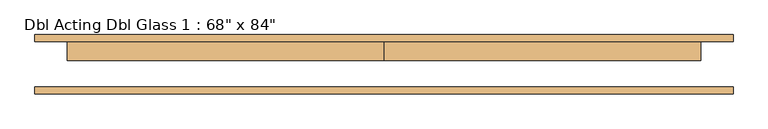
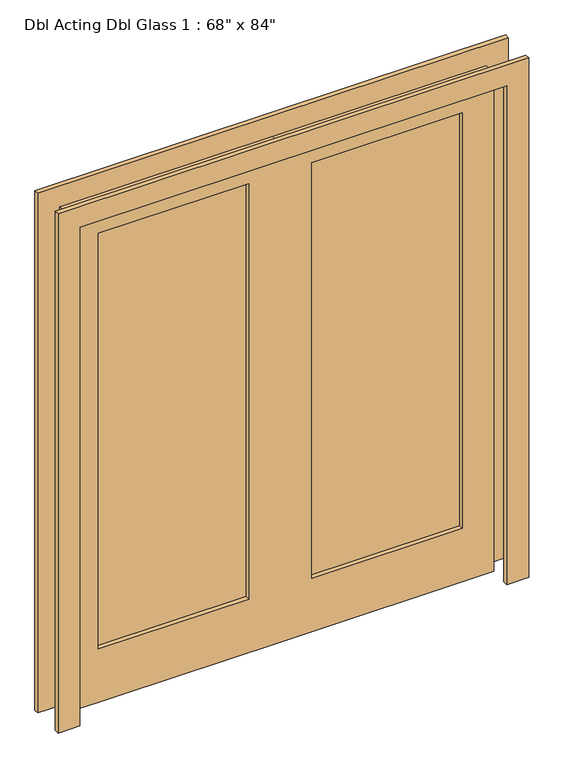
"""IFC4 building model written with IfcOpenShell, lengths in millimetres: door geometry."""

from ifc_helpers import new_model, si_unit, frame, origin, place, context, project, spatial, polyline, outline, extrude, source, transform, mapped, element, save


def door_85c6249d(model_context):
    return source(origin(), model_context, "Body", "SweptSolid", [
        extrude(outline(polyline([(127.0, 68.2625), (736.6, 68.2625), (736.6, 55.5625), (127.0, 55.5625), (127.0, 68.2625)])), frame((0.0, 0.0, 228.6), z_axis=(0.0, 0.0, 1.0), x_axis=(1.0, 0.0, 0.0)), (0.0, 0.0, 1.0), 1778.0),
        extrude(outline(polyline([(-736.6, 68.2625), (-127.0, 68.2625), (-127.0, 55.5625), (-736.6, 55.5625), (-736.6, 68.2625)])), frame((0.0, 0.0, 228.6), z_axis=(0.0, 0.0, 1.0), x_axis=(1.0, 0.0, 0.0)), (0.0, 0.0, 1.0), 1778.0),
        extrude(outline(polyline([(2133.6, 0.0), (2133.6, -863.6), (0.0, -863.6), (0.0, 0.0), (0.0, 863.6), (2133.6, 863.6), (2133.6, 0.0)]), holes=[polyline([(2006.6, 127.0), (2006.6, 736.6), (228.6, 736.6), (228.6, 127.0), (2006.6, 127.0)]), polyline([(2006.6, -127.0), (228.6, -127.0), (228.6, -736.6), (2006.6, -736.6), (2006.6, -127.0)])]), frame((0.0, 36.5125, 0.0), z_axis=(0.0, 1.0, 0.0), x_axis=(0.0, 0.0, 1.0)), (0.0, 0.0, 1.0), 50.8),
        extrude(outline(polyline([(2133.6, -863.6), (2133.6, 863.6), (0.0, 863.6), (0.0, 952.5), (2222.5, 952.5), (2222.5, -952.5), (0.0, -952.5), (0.0, -863.6), (2133.6, -863.6)])), frame((0.0, -55.5625, 0.0), z_axis=(0.0, 1.0, 0.0), x_axis=(0.0, 0.0, 1.0)), (0.0, 0.0, 1.0), 19.05),
        extrude(outline(polyline([(2133.6, -863.6), (2133.6, 863.6), (0.0, 863.6), (0.0, 952.5), (2222.5, 952.5), (2222.5, -952.5), (0.0, -952.5), (0.0, -863.6), (2133.6, -863.6)])), frame((0.0, 87.3125, 0.0), z_axis=(0.0, 1.0, 0.0), x_axis=(0.0, 0.0, 1.0)), (0.0, 0.0, 1.0), 19.05),
    ])


if __name__ == "__main__":
    model = new_model("IFC4")
    model_context = context("Model", 3, world=origin())
    ifc_project = project(units=[si_unit("LENGTHUNIT", "METRE", prefix="MILLI")], contexts=[model_context])
    site = spatial("IfcSite", under=ifc_project)
    building = spatial("IfcBuilding", under=site)
    placement = place(None, origin())
    door_shape = door_85c6249d(model_context)
    element("IfcDoor", 1, ObjectType="Dbl Acting Dbl Glass 1 : 68\" x 84\"", at=placement, inside=building, context=model_context, shape_type="MappedRepresentation", body=[
        mapped(door_shape, transform((0.0, 0.0, 0.0), x_axis=(1.0, 0.0, 0.0), y_axis=(0.0, 1.0, 0.0), z_axis=(0.0, 0.0, 1.0))),
    ])
    save(model, "model.ifc")

# Revit data of these elements
# Type "Dbl Acting Dbl Glass 1 : 68\" x 84\""
#   Type Mark = "33"
#   Door Thickness = 0' - 2"
#   Height = 7' - 0"
#   Rail Width - Base = 0' - 9"
#   Rail Width - Head = 0' - 5"
#   Stile Width - Hinge = 0' - 5"
#   Stile Width - Lock = 0' - 5"
#   Trim Projection Ext. = 0' - 0 3/4"
#   Trim Projection Int. = 0' - 0 3/4"
#   Trim Width Ext. = 0' - 3 1/2"
#   Trim Width Int. = 0' - 3 1/2"
#   Width = 5' - 8"
#   Function = 0
#   Wall Closure = (empty or 0)
# Element 1 (IfcDoor, "Dbl Acting Dbl Glass 1 : 68\" x 84\"")
#   Materials on its faces: "Glass"
# Materials
#   "Glass": class "Glass", colour RGB 0 128 192, transparency 0.75, Description = "Soda Lime Glass", Cost = 0
